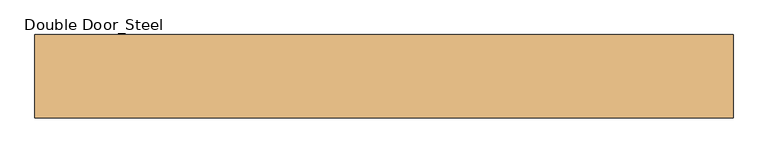
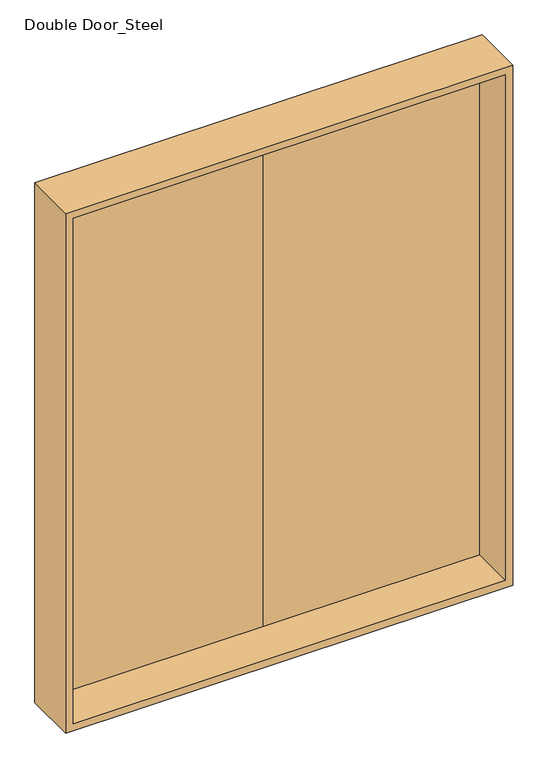
"""IFC4 building model written with IfcOpenShell, lengths in millimetres: door geometry, Double Door_Steel : H_DR_AR_B12_Double Door_Sliding_W2100xH2580_SD5."""

from ifc_helpers import new_model, si_unit, frame, origin, place, context, project, spatial, polyline, outline, extrude, faceted_brep, source, transform, mapped, element, save


def double_door_steel_dcf5a77a(model_context):
    return source(origin(), model_context, "Body", "SolidModel", [
        extrude(outline(polyline([(1030.0, 85.0), (0.0, 85.0), (0.0, 125.0), (1030.0, 125.0), (1030.0, 85.0)])), frame((0.0, 0.0, 20.0), z_axis=(0.0, 0.0, 1.0), x_axis=(1.0, 0.0, 0.0)), (0.0, 0.0, 1.0), 2540.0),
        extrude(outline(polyline([(0.0, 85.0), (-1030.0, 85.0), (-1030.0, 125.0), (0.0, 125.0), (0.0, 85.0)])), frame((0.0, 0.0, 20.0), z_axis=(0.0, 0.0, 1.0), x_axis=(1.0, 0.0, 0.0)), (0.0, 0.0, 1.0), 2540.0),
        faceted_brep([(1050.0, -125.0, 0.0), (1050.0, 125.0, 0.0), (1050.0, 125.0, 2580.0), (1050.0, -125.0, 2580.0), (-1050.0, 125.0, 2580.0), (-1050.0, -125.0, 2580.0), (-1050.0, 125.0, 0.0), (1030.0, 125.0, 2560.0), (-1030.0, 125.0, 2560.0), (-1030.0, 125.0, 20.0), (1030.0, 125.0, 20.0), (-1050.0, -125.0, 0.0), (1015.0, -125.0, 35.0), (-1015.0, -125.0, 35.0), (-1015.0, -125.0, 2545.0), (1015.0, -125.0, 2545.0), (1015.0, 85.0, 35.0), (1015.0, 85.0, 2545.0), (-1015.0, 85.0, 2545.0), (-1015.0, 85.0, 35.0), (1030.0, 85.0, 20.0), (-1030.0, 85.0, 20.0), (-1030.0, 85.0, 2560.0), (1030.0, 85.0, 2560.0)], [[[0, 1, 2, 3]], [[3, 2, 4, 5]], [[1, 6, 4, 2], [7, 8, 9, 10]], [[5, 4, 6, 11]], [[3, 5, 11, 0], [12, 13, 14, 15]], [[16, 12, 15, 17]], [[17, 15, 14, 18]], [[18, 14, 13, 19]], [[20, 21, 22, 23], [17, 18, 19, 16]], [[10, 20, 23, 7]], [[7, 23, 22, 8]], [[8, 22, 21, 9]], [[11, 6, 1, 0]], [[19, 13, 12, 16]], [[9, 21, 20, 10]]]),
    ])


if __name__ == "__main__":
    model = new_model("IFC4")
    model_context = context("Model", 3, world=origin())
    ifc_project = project(units=[si_unit("LENGTHUNIT", "METRE", prefix="MILLI")], contexts=[model_context])
    site = spatial("IfcSite", under=ifc_project)
    building = spatial("IfcBuilding", under=site)
    placement = place(None, origin())
    double_door_steel_shape = double_door_steel_dcf5a77a(model_context)
    element("IfcDoor", 1, ObjectType="Double Door_Steel : H_DR_AR_B12_Double Door_Sliding_W2100xH2580_SD5", at=placement, inside=building, context=model_context, shape_type="MappedRepresentation", body=[
        mapped(double_door_steel_shape, transform((0.0, 0.0, 0.0), x_axis=(1.0, 0.0, 0.0), y_axis=(0.0, 1.0, 0.0), z_axis=(0.0, 0.0, 1.0))),
    ])
    save(model, "model.ifc")

# Revit data of these elements
# Type "Double Door_Steel : H_DR_AR_B12_Double Door_Sliding_W2100xH2580_SD5"
#   Type Mark = "447"
#   프레임 = ""
#   철물 = ""
#   유리/마감 = ""
#   위치/개소 = ""
#   부호 = "1/SD"
#   문번호 = "5"
#   문기호 = "SD"
#   Analytic Construction = "<None>"
#   Height = 2580 mm
#   Width = 2100 mm
#   Define Thermal Properties by = 1
#   문 틀 = none
#   문 = none
#   Function = (empty or 0)
#   Assembly Code = ""
#   Wall Closure = (empty or 0)
